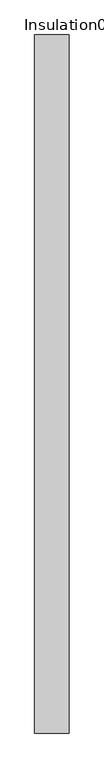
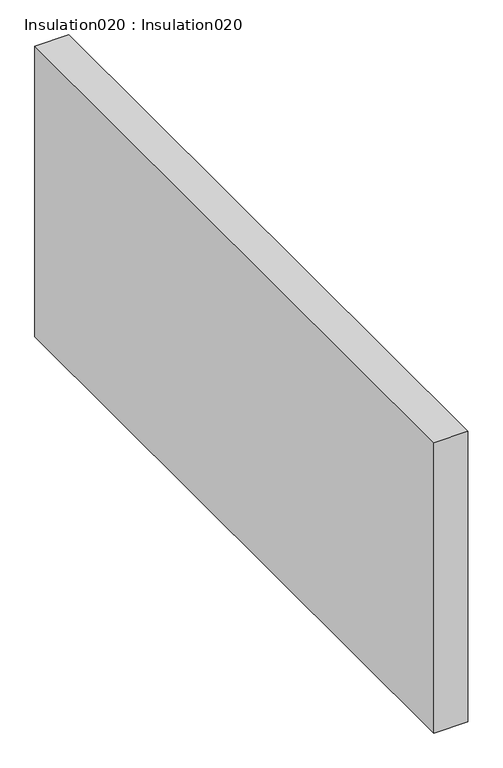
"""IFC4 building model written with IfcOpenShell, lengths in millimetres: proxy geometry, Insulation020 : Insulation020."""

from ifc_helpers import new_model, si_unit, frame, origin, place, context, project, spatial, polyline, outline, extrude, source, transform, mapped, element, save


def insulation020_insulation020_a56b5302(model_context):
    return source(origin(), model_context, "Body", "SweptSolid", [
        extrude(outline(polyline([(-9528.5644384, 7982.1526996), (-9627.1191259, 7982.1526996), (-9627.1191259, 9982.1526996), (-9528.5644384, 9982.1526996), (-9528.5644384, 7982.1526996)])), frame((0.0, 0.0, 32645.0945745), z_axis=(0.0, 0.0, 1.0), x_axis=(1.0, 0.0, 0.0)), (0.0, 0.0, 1.0), 888.999982),
    ])


if __name__ == "__main__":
    model = new_model("IFC4")
    model_context = context("Model", 3, world=origin())
    ifc_project = project(units=[si_unit("LENGTHUNIT", "METRE", prefix="MILLI")], contexts=[model_context])
    site = spatial("IfcSite", under=ifc_project)
    building = spatial("IfcBuilding", under=site)
    placement = place(None, origin())
    insulation020_insulation020_shape = insulation020_insulation020_a56b5302(model_context)
    element("IfcBuildingElementProxy", 1, Name="Insulation020 : Insulation020", ObjectType="Insulation020 : Insulation020", at=placement, inside=building, context=model_context, shape_type="MappedRepresentation", body=[
        mapped(insulation020_insulation020_shape, transform((0.0, 0.0, 0.0), x_axis=(1.0, 0.0, 0.0), y_axis=(0.0, 1.0, 0.0), z_axis=(0.0, 0.0, 1.0))),
    ])
    save(model, "model.ifc")

# Revit data of these elements
# Type "Insulation020 : Insulation020"
#   NameOverride = "Insulation020"
# Element 1 (IfcBuildingElementProxy, "Insulation020 : Insulation020")
#   Materials on its faces: "BATT INSULATION (U-FACTOR = 0.065 MIN.) OVER CLASS II VAPOR RETARDER (TOWARDS INTERIOR)"
# Materials
#   "BATT INSULATION (U-FACTOR = 0.065 MIN.) OVER CLASS II VAPOR RETARDER (TOWARDS INTERIOR)": class "Unassigned", colour RGB 246 242 160, transparency 0, Cost = 0
